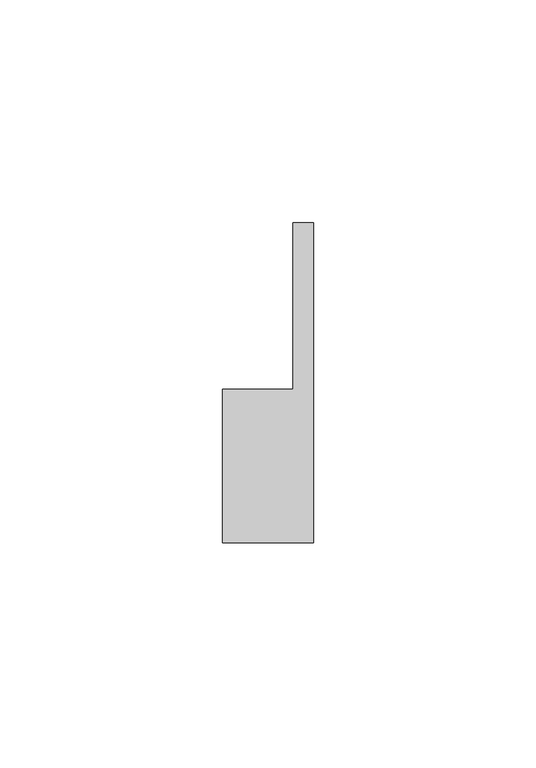
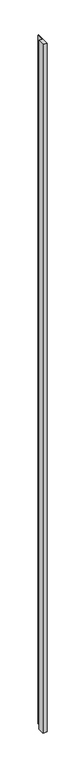
"""IFC4 building model written with IfcOpenShell, lengths in millimetres: proxy geometry, Generic Models 11:Generic Models 1:306267:Generic Models 1:306267 : Generic Models 11:Generic Models 1:306267:300405:Generic Models 1:306267:Generic Models 1:306267 : Generic Models 11:Generic Models 1:306267:300405 : Generic Models 11:Generic Models 1:306267:Generic Models 1:306267 : Generic Models 11:Generic Models 1:306267:300405:3 : Generic Models 11:Generic Models 1:306267:Generic Models 1:306267 : Generic Models 11:Generic Models 1:306267:300405:Generic Models 1:306267:Generic Models 1:306267 : Generic Models 11:Generic Models 1:306267:300405 : Generic Models 11:Generic Models 1:306267:Generic Models 1:306267 : Generic Models 11:Generic Models 1:306267:300405:300182."""

import ifcopenshell
import ifcopenshell.guid

model = None  # the IFC model being written
_history = None  # IfcOwnerHistory: only IFC2X3 demands one
_inside = {}  # id of a spatial element -> (the spatial element, [elements in it])
_under = {}  # id of a project, library or spatial element -> (it, [spatial elements below it])
_declared = {}  # id of a project -> (the project, [libraries it declares])
_typed = {}  # id of a type object -> (the type object, [elements of that type])
_made_of = {}  # id of a material, layer set ... -> (it, [elements and type objects made of it])


def new_model(schema):
    """Start an empty IFC model of exactly this schema.

    Asked for "IFC4X3", IfcOpenShell would pick the latest addendum, in which some entities
    have other attributes; the version numbers below select the first issue.
    IFC2X3 requires an IfcOwnerHistory on every rooted entity: one is made here for all.
    """
    global model, _history
    if schema == "IFC4X3":
        model = ifcopenshell.file(schema_version=(4, 3, 0, 0))
    else:
        model = ifcopenshell.file(schema=schema)
    _inside.clear()
    _under.clear()
    _declared.clear()
    _typed.clear()
    _made_of.clear()
    _history = None
    if model.schema == "IFC2X3":
        org = make("IfcOrganization", Name="unknown")
        user = make(
            "IfcPersonAndOrganization",
            ThePerson=make("IfcPerson", FamilyName="unknown"),
            TheOrganization=org,
        )
        app = make(
            "IfcApplication",
            ApplicationDeveloper=org,
            Version="unknown",
            ApplicationFullName="unknown",
            ApplicationIdentifier="unknown",
        )
        _history = make(
            "IfcOwnerHistory",
            OwningUser=user,
            OwningApplication=app,
            ChangeAction="ADDED",
            CreationDate=0,
        )
    return model


def make(cls, **values):
    """One entity of the class cls with the attributes given. An attribute that is None is left unset."""
    return model.create_entity(
        cls, **{name: value for name, value in values.items() if value is not None}
    )


def rooted(cls, **values):
    """An entity with a GlobalId (a new one), such as an element, a storey or a relation."""
    return make(cls, GlobalId=ifcopenshell.guid.new(), OwnerHistory=_history, **values)


def si_unit(unit_type, name, prefix=None):
    """IfcSIUnit, for example si_unit("LENGTHUNIT", "METRE", prefix="MILLI")."""
    return make("IfcSIUnit", UnitType=unit_type, Prefix=prefix, Name=name)


def assignment(units):
    """IfcUnitAssignment: the units of a project."""
    return None if units is None else make("IfcUnitAssignment", Units=units)


def point(xyz):
    """IfcCartesianPoint."""
    return None if xyz is None else make("IfcCartesianPoint", Coordinates=xyz)


def direction(xyz):
    """IfcDirection."""
    return None if xyz is None else make("IfcDirection", DirectionRatios=xyz)


def frame(location, z_axis=None, x_axis=None):
    """IfcAxis2Placement3D, a coordinate frame: its origin and axes. An axis left out is left unset."""
    return make(
        "IfcAxis2Placement3D",
        Location=point(location),
        Axis=direction(z_axis),
        RefDirection=direction(x_axis),
    )


def origin():
    """The frame at (0, 0, 0) with its axes left unset."""
    return frame((0.0, 0.0, 0.0))


def origin_with_axes():
    """The frame at (0, 0, 0) with the z axis (0, 0, 1) and the x axis (1, 0, 0) written out."""
    return frame((0.0, 0.0, 0.0), z_axis=(0.0, 0.0, 1.0), x_axis=(1.0, 0.0, 0.0))


def place(relative_to, where):
    """IfcLocalPlacement: puts the frame where relative to a parent placement (None: the world)."""
    return make(
        "IfcLocalPlacement", PlacementRelTo=relative_to, RelativePlacement=where
    )


def context(
    kind, dimensions, precision=None, world=None, true_north=None, identifier=None
):
    """IfcGeometricRepresentationContext, for example the 3D "Model" context."""
    return make(
        "IfcGeometricRepresentationContext",
        ContextIdentifier=identifier,
        ContextType=kind,
        CoordinateSpaceDimension=dimensions,
        Precision=precision,
        WorldCoordinateSystem=world,
        TrueNorth=true_north,
    )


def project(units=None, contexts=None):
    """IfcProject with its units and contexts."""
    return rooted(
        "IfcProject",
        Name="project",
        RepresentationContexts=contexts,
        UnitsInContext=assignment(units),
    )


def spatial(cls, under=None, at=None, **own):
    """A site, building, storey or space (cls), placed at a placement, below another one or the project."""
    s = rooted(cls, ObjectPlacement=at, **own)
    if under is not None:
        _under.setdefault(under.id(), (under, []))[1].append(s)
    return s


def polyline(points):
    """IfcPolyline through the points."""
    return make("IfcPolyline", Points=[point(p) for p in points])


def outline(outer, holes=None, kind="AREA"):
    """IfcArbitraryClosedProfileDef: a profile drawn as a closed curve; with holes, ...WithVoids."""
    if holes is None:
        return make("IfcArbitraryClosedProfileDef", ProfileType=kind, OuterCurve=outer)
    return make(
        "IfcArbitraryProfileDefWithVoids",
        ProfileType=kind,
        OuterCurve=outer,
        InnerCurves=holes,
    )


def extrude(swept, where, along, depth):
    """IfcExtrudedAreaSolid: the profile swept, set in the frame where, extruded along a direction by depth."""
    return make(
        "IfcExtrudedAreaSolid",
        SweptArea=swept,
        Position=where,
        ExtrudedDirection=direction(along),
        Depth=depth,
    )


def shape(context_of_items, identifier, shape_type, items):
    """IfcShapeRepresentation: the items that make up one representation, for example the "Body"."""
    return make(
        "IfcShapeRepresentation",
        ContextOfItems=context_of_items,
        RepresentationIdentifier=identifier,
        RepresentationType=shape_type,
        Items=items,
    )


def source(mapping_origin, context_of_items, identifier, shape_type, items):
    """IfcRepresentationMap: a shape defined once, which mapped items show again and again."""
    return make(
        "IfcRepresentationMap",
        MappingOrigin=mapping_origin,
        MappedRepresentation=shape(context_of_items, identifier, shape_type, items),
    )


def transform(
    local_origin,
    x_axis=None,
    y_axis=None,
    z_axis=None,
    scale=None,
    scale2=None,
    scale3=None,
    uniform=True,
):
    """IfcCartesianTransformationOperator3D, or its non-uniform kind. x_axis, y_axis, z_axis: its Axis1, 2, 3."""
    if uniform:
        return make(
            "IfcCartesianTransformationOperator3D",
            Axis1=direction(x_axis),
            Axis2=direction(y_axis),
            LocalOrigin=point(local_origin),
            Scale=scale,
            Axis3=direction(z_axis),
        )
    return make(
        "IfcCartesianTransformationOperator3DnonUniform",
        Axis1=direction(x_axis),
        Axis2=direction(y_axis),
        LocalOrigin=point(local_origin),
        Scale=scale,
        Axis3=direction(z_axis),
        Scale2=scale2,
        Scale3=scale3,
    )


def mapped(mapping_source, mapping_target):
    """IfcMappedItem: shows the shape of a source again, moved by a transform."""
    return make(
        "IfcMappedItem", MappingSource=mapping_source, MappingTarget=mapping_target
    )


def made_of(thing, what):
    """Note that an element or type object is made of a material, layer set ...; save() writes the relation."""
    if what is not None:
        _made_of.setdefault(what.id(), (what, []))[1].append(thing)
    return thing


def element(
    cls,
    number,
    at=None,
    inside=None,
    cuts=None,
    type_object=None,
    material=None,
    context=None,
    identifier="Body",
    shape_type=None,
    held_by="IfcProductDefinitionShape",
    body=None,
    shapes=None,
    **own,
):
    """One element of the class cls, such as IfcWall. Its Tag is "e" and its number.

    at: its placement. inside: the storey or other place that contains it. cuts: it is an
    opening in that element (IfcRelVoidsElement). A single representation is given by context,
    identifier, shape_type and body (its items); several are given by shapes. held_by: the class
    of the entity that holds the representations. save() writes the other relations.
    """
    e = rooted(cls, Tag="e%d" % number, ObjectPlacement=at, **own)
    if body is not None:
        shapes = [shape(context, identifier, shape_type, body)]
    if shapes is not None:
        e.Representation = make(held_by, Representations=shapes)
    if inside is not None:
        _inside.setdefault(inside.id(), (inside, []))[1].append(e)
    if cuts is not None:
        rooted(
            "IfcRelVoidsElement", RelatingBuildingElement=cuts, RelatedOpeningElement=e
        )
    if type_object is not None:
        _typed.setdefault(type_object.id(), (type_object, []))[1].append(e)
    return made_of(e, material)


def aggregate(whole, parts):
    """IfcRelAggregates: a whole, such as a stair, and the parts it consists of."""
    return rooted("IfcRelAggregates", RelatingObject=whole, RelatedObjects=parts)


def save(model, path):
    """Write the relations noted so far, then the file.

    IfcRelAggregates (storeys below a building ...), IfcRelContainedInSpatialStructure (elements
    in a storey), IfcRelDefinesByType, IfcRelAssociatesMaterial and IfcRelDeclares: one each for
    every whole, place, type object, material and project.
    """
    for whole, parts in _under.values():
        aggregate(whole, parts)
    for where, things in _inside.values():
        rooted(
            "IfcRelContainedInSpatialStructure",
            RelatedElements=things,
            RelatingStructure=where,
        )
    for kind, things in _typed.values():
        rooted("IfcRelDefinesByType", RelatedObjects=things, RelatingType=kind)
    for what, things in _made_of.values():
        rooted("IfcRelAssociatesMaterial", RelatedObjects=things, RelatingMaterial=what)
    for by, libraries in _declared.values():
        rooted("IfcRelDeclares", RelatingContext=by, RelatedDefinitions=libraries)
    model.write(path)


def generic_models_83a68f1d(model_context):
    return source(origin(), model_context, "Body", "SweptSolid", [
        extrude(outline(polyline([(593732.6688081, -579043.9402916), (593732.6688081, -579006.5153982), (593737.3091519, -579006.5153982), (593737.3091519, -579078.4496134), (593716.7987584, -579078.4496134), (593716.7987584, -579043.9402916), (593732.6688081, -579043.9402916)])), origin_with_axes(), (0.0, 0.0, 1.0), 3689.35),
    ])


if __name__ == "__main__":
    model = new_model("IFC4")
    model_context = context("Model", 3, world=origin())
    ifc_project = project(units=[si_unit("LENGTHUNIT", "METRE", prefix="MILLI")], contexts=[model_context])
    site = spatial("IfcSite", under=ifc_project)
    building = spatial("IfcBuilding", under=site)
    placement = place(None, origin())
    generic_models_shape = generic_models_83a68f1d(model_context)
    element("IfcBuildingElementProxy", 1, Name="Generic Models 11:Generic Models 1:306267:Generic Models 1:306267 : Generic Models 11:Generic Models 1:306267:300405:Generic Models 1:306267:Generic Models 1:306267 : Generic Models 11:Generic Models 1:306267:300405 : Generic Models 11:Generic Models 1:306267:Generic Models 1:306267 : Generic Models 11:Generic Models 1:306267:300405:3 : Generic Models 11:Generic Models 1:306267:Generic Models 1:306267 : Generic Models 11:Generic Models 1:306267:300405:Generic Models 1:306267:Generic Models 1:306267 : Generic Models 11:Generic Models 1:306267:300405 : Generic Models 11:Generic Models 1:306267:Generic Models 1:306267 : Generic Models 11:Generic Models 1:306267:300405:300182", ObjectType="Generic Models 11:Generic Models 1:306267:Generic Models 1:306267 : Generic Models 11:Generic Models 1:306267:300405:Generic Models 1:306267:Generic Models 1:306267 : Generic Models 11:Generic Models 1:306267:300405 : Generic Models 11:Generic Models 1:306267:Generic Models 1:306267 : Generic Models 11:Generic Models 1:306267:300405:3 : Generic Models 11:Generic Models 1:306267:Generic Models 1:306267 : Generic Models 11:Generic Models 1:306267:300405:Generic Models 1:306267:Generic Models 1:306267 : Generic Models 11:Generic Models 1:306267:300405 : Generic Models 11:Generic Models 1:306267:Generic Models 1:306267 : Generic Models 11:Generic Models 1:306267:300405:300182", at=placement, inside=building, context=model_context, shape_type="MappedRepresentation", body=[
        mapped(generic_models_shape, transform((0.0, 0.0, 0.0), x_axis=(1.0, 0.0, 0.0), y_axis=(0.0, 1.0, 0.0), z_axis=(0.0, 0.0, 1.0))),
    ])
    save(model, "model.ifc")

# Revit data of these elements
# Type "Generic Models 11:Generic Models 1:306267:Generic Models 1:306267 : Generic Models 11:Generic Models 1:306267:300405:Generic Models 1:306267:Generic Models 1:306267 : Generic Models 11:Generic Models 1:306267:300405 : Generic Models 11:Generic Models 1:306267:Generic Models 1:306267 : Generic Models 11:Generic Models 1:306267:300405:3 : Generic Models 11:Generic Models 1:306267:Generic Models 1:306267 : Generic Models 11:Generic Models 1:306267:300405:Generic Models 1:306267:Generic Models 1:306267 : Generic Models 11:Generic Models 1:306267:300405 : Generic Models 11:Generic Models 1:306267:Generic Models 1:306267 : Generic Models 11:Generic Models 1:306267:300405:300182"
#   NameOverride = "Generic Models 11:Generic Models 1:306267:Generic Models 1:306267 : Generic Models 11:Generic Models 1:306267:300405:Generic Models 1:306267:Generic Models 1:306267 : Generic Models 11:Generic Models 1:306267:300405 : Generic Models 11:Generic Models 1:306267:Generic Models 1:306267 : Generic Models 11:Generic Models 1:306267:300405:300182"
#   ObjectTypeOverride = "Generic Models 1:306267:Generic Models 1:306267 : Generic Models 11:Generic Models 1:306267:300405 : Generic Models 11:Generic Models 1:306267:Generic Models 1:306267 : Generic Models 11:Generic Models 1:306267:300405"
#   Reference = "Generic Models 1"
#   Tag = "300182"
# Element 1 (IfcBuildingElementProxy, "Generic Models 11:Generic Models 1:306267:Generic Models 1:306267 : Generic Models 11:Generic Models 1:306267:300405:Generic Models 1:306267:Generic Models 1:306267 : Generic Models 11:Generic Models 1:306267:300405 : Generic Models 11:Generic Models 1:306267:Generic Models 1:306267 : Generic Models 11:Generic Models 1:306267:300405:3 : Generic Models 11:Generic Models 1:306267:Generic Models 1:306267 : Generic Models 11:Generic Models 1:306267:300405:Generic Models 1:306267:Generic Models 1:306267 : Generic Models 11:Generic Models 1:306267:300405 : Generic Models 11:Generic Models 1:306267:Generic Models 1:306267 : Generic Models 11:Generic Models 1:306267:300405:300182")
#   Materials on its faces: "LOW VOLUMN EXPANDABLE FOAM INSULATION"
# Materials
#   "LOW VOLUMN EXPANDABLE FOAM INSULATION": class "Unassigned", colour RGB 213 216 95, transparency 0, Cost = 0
